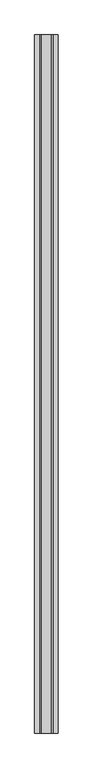
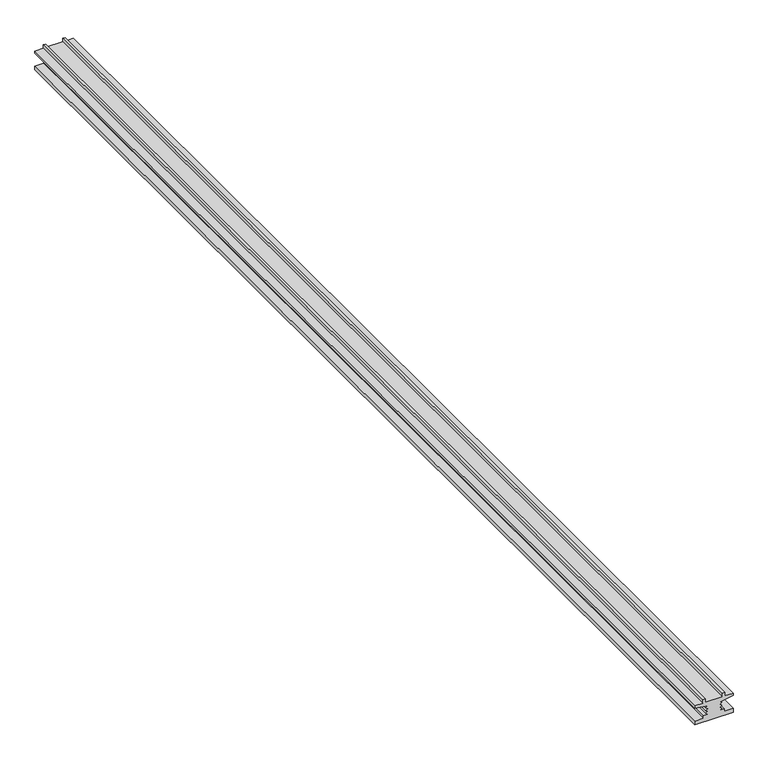
"""IFC4 building model written with IfcOpenShell, lengths in millimetres: proxy geometry, Bison pedestal2:Bison pedestal005:295399 : Bison pedestal2:Bison pedestal005:295399."""

from ifc_helpers import new_model, si_unit, frame, origin, place, context, project, spatial, polyline, outline, extrude, source, transform, mapped, element, save


def generic_models_332994b9(model_context):
    return source(origin(), model_context, "Body", "SweptSolid", [
        extrude(outline(polyline([(36480.0342739, 2545.3209848), (36480.0342739, 2612.7416648), (36486.734375, 2612.8062271), (36486.734375, 2597.3867935), (36491.2120625, 2597.3867935), (36491.2120625, 2589.2957291), (36494.1534687, 2592.8264908), (36496.7296406, 2589.5164322), (36499.4503437, 2593.0469498), (36502.0245625, 2589.6634049), (36504.5577656, 2593.2381119), (36507.1046406, 2590.0215592), (36510.9913594, 2612.8062271), (36515.1456562, 2612.8062271), (36515.1456562, 2598.0630631), (36521.3116719, 2598.0630631), (36521.3116719, 2594.1763443), (36515.1456562, 2594.1763443), (36515.1456562, 2563.8863053), (36521.3116719, 2563.8863053), (36521.3116719, 2559.9995865), (36515.1456562, 2559.9995865), (36515.1456562, 2545.2564224), (36510.9913594, 2545.2564224), (36507.1046406, 2568.0410904), (36504.5577656, 2564.8245377), (36502.0245625, 2568.3992447), (36499.4503437, 2565.0156998), (36496.7296406, 2568.5462174), (36494.1534687, 2565.2361588), (36491.2120625, 2568.7669205), (36491.2120625, 2560.675856), (36486.734375, 2560.675856), (36486.734375, 2545.2564224), (36480.0342739, 2545.3209848)])), frame((0.0, 1276.4895464, 0.0), z_axis=(0.0, 1.0, 0.0), x_axis=(0.0, 0.0, 1.0)), (0.0, 0.0, 1.0), 2000.0),
    ])


if __name__ == "__main__":
    model = new_model("IFC4")
    model_context = context("Model", 3, world=origin())
    ifc_project = project(units=[si_unit("LENGTHUNIT", "METRE", prefix="MILLI")], contexts=[model_context])
    site = spatial("IfcSite", under=ifc_project)
    building = spatial("IfcBuilding", under=site)
    placement = place(None, origin())
    generic_models_shape = generic_models_332994b9(model_context)
    element("IfcBuildingElementProxy", 1, Name="Bison pedestal2:Bison pedestal005:295399 : Bison pedestal2:Bison pedestal005:295399", ObjectType="Bison pedestal2:Bison pedestal005:295399 : Bison pedestal2:Bison pedestal005:295399", at=placement, inside=building, context=model_context, shape_type="MappedRepresentation", body=[
        mapped(generic_models_shape, transform((0.0, 0.0, 0.0), x_axis=(1.0, 0.0, 0.0), y_axis=(0.0, 1.0, 0.0), z_axis=(0.0, 0.0, 1.0))),
    ])
    save(model, "model.ifc")

# Revit data of these elements
# Type "Bison pedestal2:Bison pedestal005:295399 : Bison pedestal2:Bison pedestal005:295399"
#   NameOverride = "Bison pedestal2:Bison pedestal005:295399"
#   ObjectTypeOverride = "Bison pedestal2:Bison pedestal005"
#   Reference = "Bison pedestal005"
#   Category = "Generic Models"
#   Tag = "295399"
# Element 1 (IfcBuildingElementProxy, "Bison pedestal2:Bison pedestal005:295399 : Bison pedestal2:Bison pedestal005:295399")
#   Materials on its faces: "BUZON PEDESTAL"
# Materials
#   "BUZON PEDESTAL": class "Unassigned", colour RGB 66 66 66, transparency 0
